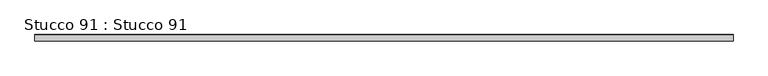
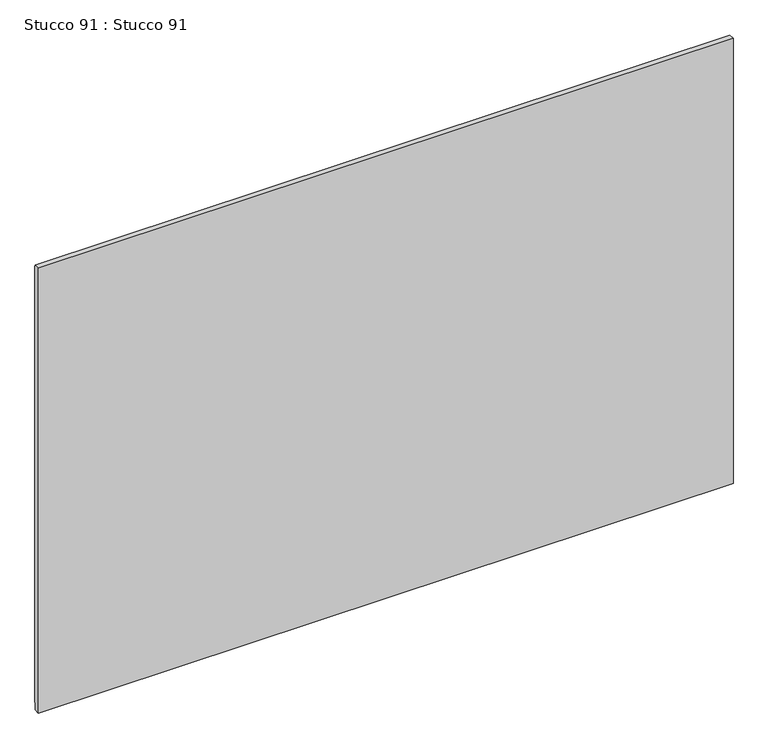
"""IFC4 building model written with IfcOpenShell, lengths in millimetres: proxy geometry, Stucco 91 : Stucco 91."""

from ifc_helpers import new_model, si_unit, frame, origin, place, context, project, spatial, polyline, outline, extrude, source, transform, mapped, element, save


def stucco_91_stucco_91_bd241f2d(model_context):
    return source(origin(), model_context, "Body", "SweptSolid", [
        extrude(outline(polyline([(10462.1750834, 39425.2967615), (10460.8950834, 39425.2967615), (10460.8950834, 39402.766), (10444.3950834, 39402.766), (10444.3950834, 40757.6682813), (10460.9050834, 40757.6682813), (10460.9050834, 40754.1884813), (10462.1750834, 40754.1884813), (10462.1750834, 39425.2967615)])), frame((3694.2883192, 0.0, 0.0), z_axis=(1.0, 0.0, 0.0), x_axis=(0.0, 1.0, 0.0)), (0.0, 0.0, 1.0), 2000.0),
    ])


if __name__ == "__main__":
    model = new_model("IFC4")
    model_context = context("Model", 3, world=origin())
    ifc_project = project(units=[si_unit("LENGTHUNIT", "METRE", prefix="MILLI")], contexts=[model_context])
    site = spatial("IfcSite", under=ifc_project)
    building = spatial("IfcBuilding", under=site)
    placement = place(None, origin())
    stucco_91_stucco_91_shape = stucco_91_stucco_91_bd241f2d(model_context)
    element("IfcBuildingElementProxy", 1, Name="Stucco 91 : Stucco 91", ObjectType="Stucco 91 : Stucco 91", at=placement, inside=building, context=model_context, shape_type="MappedRepresentation", body=[
        mapped(stucco_91_stucco_91_shape, transform((0.0, 0.0, 0.0), x_axis=(1.0, 0.0, 0.0), y_axis=(0.0, 1.0, 0.0), z_axis=(0.0, 0.0, 1.0))),
    ])
    save(model, "model.ifc")

# Revit data of these elements
# Type "Stucco 91 : Stucco 91"
#   NameOverride = "Stucco"
# Element 1 (IfcBuildingElementProxy, "Stucco 91 : Stucco 91")
#   Materials on its faces: "7/8\" SMOOTH TROWEL EXTERIOR STUCCO"
# Materials
#   "7/8\" SMOOTH TROWEL EXTERIOR STUCCO": class "Unassigned", colour RGB 255 255 255, transparency 0, Cost = 0
